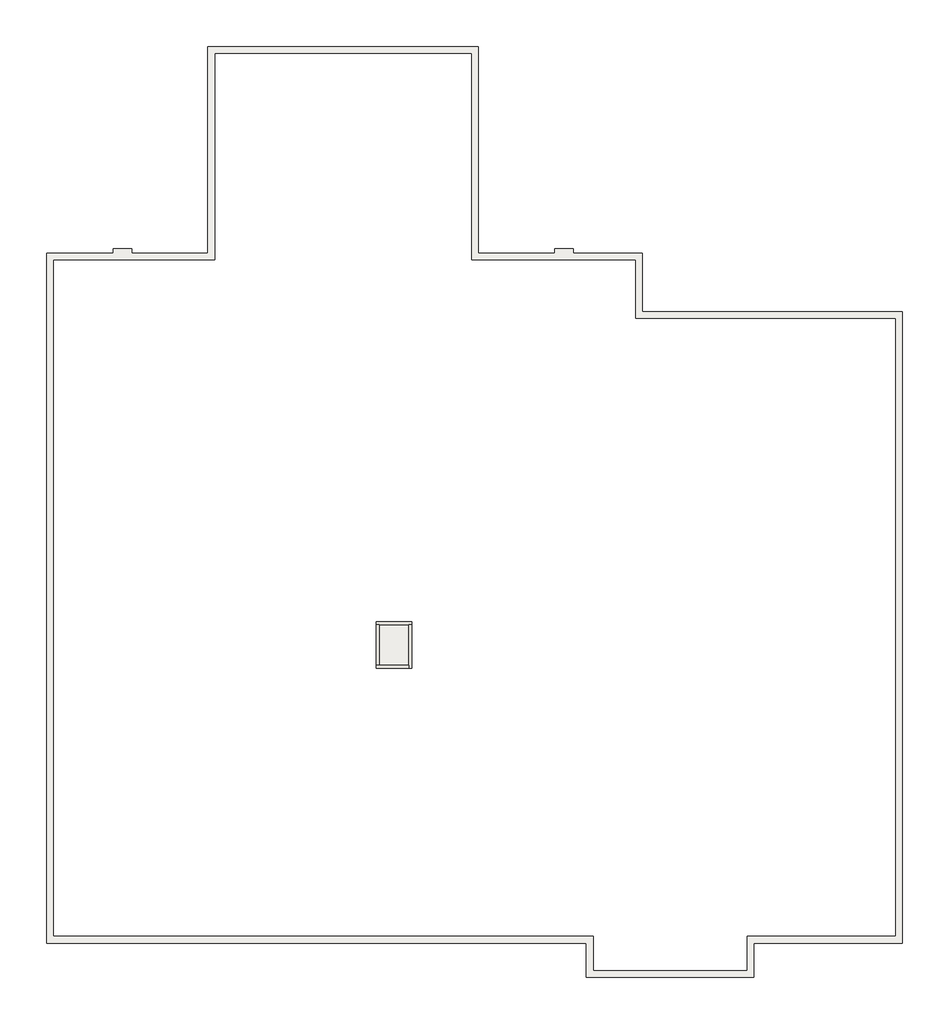
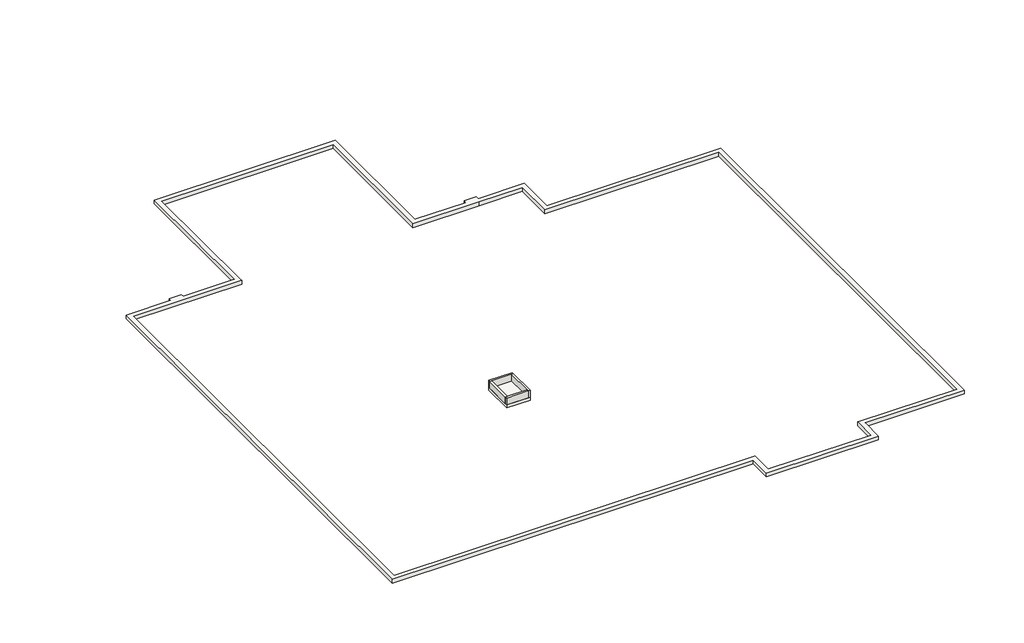
# One storey: 4 walls, 2 slabs.
# Revit data of these elements (continued)
# Project information (continued)
#   PrintManagerSettings = "<PrintManagerDS xmlns=\"http://tempuri.org/PrintManagerDS.xsd\">\n  <xs:schema id=\"PrintManagerDS\" targetNamespace=\"http://tempuri.org/PrintManagerDS.xsd\" xmlns:mstns=\"http://tempuri.org/PrintManagerDS.xsd\" xmlns=\"http://tempuri.org/PrintManagerDS.xsd\" xmlns:xs=\"http://www.w3.org/2001/XMLSchema\" xmlns:msdata=\"urn:schemas-microsoft-com:xml-msdata\" attributeFormDefault=\"qualified\" elementFormDefault=\"qualified\">\n    <xs:element name=\"PrintManagerDS\" msdata:IsDataSet=\"true\" msdata:UseCurrentLocale=\"true\">\n      <xs:complexType>\n        <xs:choice minOccurs=\"0\" maxOccurs=\"unbounded\">\n          <xs:element name=\"DruckEinstellungDT\">\n            <xs:complexType>\n              <xs:sequence>\n                <xs:element name=\"ID\" msdata:DataType=\"System.Guid, mscorlib, Version=4.0.0.0, Culture=neutral, PublicKeyToken=b77a5c561934e089\" msdata:AutoIncrementSeed=\"-1\" msdata:AutoIncrementStep=\"-1\" type=\"xs:string\" minOccurs=\"0\" />\n                <xs:element name=\"Name\" type=\"xs:string\" minOccurs=\"0\" />\n                <xs:element name=\"Beschreibung\" type=\"xs:string\" minOccurs=\"0\" />\n                <xs:element name=\"Kategorie\" type=\"xs:string\" minOccurs=\"0\" />\n                <xs:element name=\"PrinterName\" type=\"xs:string\" minOccurs=\"0\" />\n                <xs:element name=\"PrintToFile\" type=\"xs:boolean\" minOccurs=\"0\" />\n                <xs:element name=\"FileName\" type=\"xs:string\" minOccurs=\"0\" />\n                <xs:element name=\"ColorDepth\" type=\"xs:string\" minOccurs=\"0\" />\n                <xs:element name=\"HiddenLineViews\" type=\"xs:string\" minOccurs=\"0\" />\n                <xs:element name=\"HideCropBoundaries\" type=\"xs:boolean\" minOccurs=\"0\" />\n                <xs:element name=\"HideRefOrWorkPlanes\" type=\"xs:boolean\" minOccurs=\"0\" />\n                <xs:element name=\"HideScopeBoxes\" type=\"xs:boolean\" minOccurs=\"0\" />\n                <xs:element name=\"HideUnreferencedViewTags\" type=\"xs:boolean\" minOccurs=\"0\" />\n                <xs:element name=\"MarginType\" type=\"xs:string\" minOccurs=\"0\" />\n                <xs:element name=\"PageOrientation\" type=\"xs:string\" minOccurs=\"0\" />\n                <xs:element name=\"PaperPlacement\" type=\"xs:string\" minOccurs=\"0\" />\n                <xs:element name=\"PaperSize\" type=\"xs:string\" minOccurs=\"0\" />\n                <xs:element name=\"PaperSource\" type=\"xs:string\" minOccurs=\"0\" />\n                <xs:element name=\"RasterQuality\" type=\"xs:string\" minOccurs=\"0\" />\n                <xs:element name=\"ReplaceHalftoneWithThinLines\" type=\"xs:boolean\" minOccurs=\"0\" />\n                <xs:element name=\"UserDefinedMarginX\" type=\"xs:double\" minOccurs=\"0\" />\n                <xs:element name=\"UserDefinedMarginY\" type=\"xs:double\" minOccurs=\"0\" />\n                <xs:element name=\"ViewLinksInBlue\" type=\"xs:boolean\" minOccurs=\"0\" />\n                <xs:element name=\"Zoom\" type=\"xs:int\" minOccurs=\"0\" />\n                <xs:element name=\"ZoomType\" type=\"xs:string\" minOccurs=\"0\" />\n              </xs:sequence>\n            </xs:complexType>\n          </xs:element>\n          <xs:element name=\"DruckSatzDT\">\n            <xs:complexType>\n              <xs:sequence>\n                <xs:element name=\"ID\" msdata:DataType=\"System.Guid, mscorlib, Version=4.0.0.0, Culture=neutral, PublicKeyToken=b77a5c561934e089\" type=\"xs:string\" minOccurs=\"0\" />\n                <xs:element name=\"PlanID\" type=\"xs:string\" minOccurs=\"0\" />\n                <xs:element name=\"DruckEinstellungID\" msdata:DataType=\"System.Guid, mscorlib, Version=4.0.0.0, Culture=neutral, PublicKeyToken=b77a5c561934e089\" type=\"xs:string\" minOccurs=\"0\" />\n                <xs:element name=\"Name\" type=\"xs:string\" minOccurs=\"0\" />\n                <xs:element name=\"Beschreibung\" type=\"xs:string\" minOccurs=\"0\" />\n                <xs:element name=\"ParameterName\" type=\"xs:string\" minOccurs=\"0\" />\n                <xs:element name=\"File\" type=\"xs:string\" minOccurs=\"0\" />\n                <xs:element name=\"Path\" type=\"xs:string\" minOccurs=\"0\" />\n                <xs:element name=\"GenerateFileName\" type=\"xs:boolean\" minOccurs=\"0\" />\n                <xs:element name=\"Kategorie\" type=\"xs:string\" minOccurs=\"0\" />\n              </xs:sequence>\n            </xs:complexType>\n          </xs:element>\n          <xs:element name=\"DruckJobDT\">\n            <xs:complexType>\n              <xs:sequence>\n                <xs:element name=\"ID\" msdata:DataType=\"System.Guid, mscorlib, Version=4.0.0.0, Culture=neutral, PublicKeyToken=b77a5c561934e089\" type=\"xs:string\" minOccurs=\"0\" />\n                <xs:element name=\"DruckJobGruppeID\" msdata:DataType=\"System.Guid, mscorlib, Version=4.0.0.0, Culture=neutral, PublicKeyToken=b77a5c561934e089\" type=\"xs:string\" minOccurs=\"0\" />\n                <xs:element name=\"DruckSatzID\" msdata:DataType=\"System.Guid, mscorlib, Version=4.0.0.0, Culture=neutral, PublicKeyToken=b77a5c561934e089\" type=\"xs:string\" minOccurs=\"0\" />\n                <xs:element name=\"Anzahl\" type=\"xs:int\" minOccurs=\"0\" />\n              </xs:sequence>\n            </xs:complexType>\n          </xs:element>\n          <xs:element name=\"DruckJobGruppeDT\">\n            <xs:complexType>\n              <xs:sequence>\n                <xs:element name=\"ID\" msdata:DataType=\"System.Guid, mscorlib, Version=4.0.0.0, Culture=neutral, PublicKeyToken=b77a5c561934e089\" type=\"xs:string\" minOccurs=\"0\" />\n                <xs:element name=\"Name\" type=\"xs:string\" minOccurs=\"0\" />\n                <xs:element name=\"Beschreibung\" type=\"xs:string\" minOccurs=\"0\" />\n                <xs:element name=\"JobCount\" msdata:ReadOnly=\"true\" msdata:Expression=\"Count(Child(DruckJobGruppeDT_DruckJobDT).Anzahl)\" type=\"xs:int\" minOccurs=\"0\" />\n                <xs:element name=\"Kategorie\" type=\"xs:string\" minOccurs=\"0\" />\n              </xs:sequence>\n            </xs:complexType>\n          </xs:element>\n          <xs:element name=\"PrintSettingCategories\">\n            <xs:complexType>\n              <xs:sequence>\n                <xs:element name=\"CategoryName\" type=\"xs:string\" minOccurs=\"0\" />\n              </xs:sequence>\n            </xs:complexType>\n          </xs:element>\n          <xs:element name=\"PrintRecordCategories\">\n            <xs:complexType>\n              <xs:sequence>\n                <xs:element name=\"CategoryName\" type=\"xs:string\" />\n              </xs:sequence>\n            </xs:complexType>\n          </xs:element>\n          <xs:element name=\"JobGroupCategories\">\n            <xs:complexType>\n              <xs:sequence>\n                <xs:element name=\"CategoryName\" type=\"xs:string\" />\n              </xs:sequence>\n            </xs:complexType>\n          </xs:element>\n          <xs:element name=\"ExportSettingsDT\">\n            <xs:complexType>\n              <xs:sequence>\n                <xs:element name=\"ID\" msdata:DataType=\"System.Guid, mscorlib, Version=4.0.0.0, Culture=neutral, PublicKeyToken=b77a5c561934e089\" type=\"xs:string\" />\n                <xs:element name=\"Name\" type=\"xs:string\" minOccurs=\"0\" />\n                <xs:element name=\"Description\" type=\"xs:string\" default=\"&quot;&quot;\" minOccurs=\"0\" />\n                <xs:element name=\"Category\" type=\"xs:string\" minOccurs=\"0\" />\n                <xs:element name=\"Type\" type=\"xs:string\" minOccurs=\"0\" />\n                <xs:element name=\"Data\" type=\"xs:string\" minOccurs=\"0\" />\n              </xs:sequence>\n            </xs:complexType>\n          </xs:element>\n          <xs:element name=\"ExportMappingDT\">\n            <xs:complexType>\n              <xs:sequence>\n                <xs:element name=\"ID\" msdata:DataType=\"System.Guid, mscorlib, Version=4.0.0.0, Culture=neutral, PublicKeyToken=b77a5c561934e089\" type=\"xs:string\" />\n                <xs:element name=\"DWG\" msdata:DataType=\"System.Guid, mscorlib, Version=4.0.0.0, Culture=neutral, PublicKeyToken=b77a5c561934e089\" type=\"xs:string\" minOccurs=\"0\" />\n                <xs:element name=\"DWGPath\" type=\"xs:string\" minOccurs=\"0\" />\n                <xs:element name=\"DWGFile\" type=\"xs:string\" minOccurs=\"0\" />\n              </xs:sequence>\n            </xs:complexType>\n          </xs:element>\n          <xs:element name=\"ExportSettingCategories\">\n            <xs:complexType>\n              <xs:sequence>\n                <xs:element name=\"CategoryName\" type=\"xs:string\" />\n              </xs:sequence>\n            </xs:complexType>\n          </xs:element>\n        </xs:choice>\n      </xs:complexType>\n      <xs:unique name=\"Constraint1\">\n        <xs:selector xpath=\".//mstns:DruckEinstellungDT\" />\n        <xs:field xpath=\"mstns:ID\" />\n      </xs:unique>\n      <xs:unique name=\"Constraint2\">\n        <xs:selector xpath=\".//mstns:DruckEinstellungDT\" />\n        <xs:field xpath=\"mstns:Name\" />\n      </xs:unique>\n      <xs:unique name=\"DruckSatzDT_Constraint1\" msdata:ConstraintName=\"Constraint1\">\n        <xs:selector xpath=\".//mstns:DruckSatzDT\" />\n        <xs:field xpath=\"mstns:ID\" />\n      </xs:unique>\n      <xs:unique name=\"DruckJobDT_Constraint1\" msdata:ConstraintName=\"Constraint1\">\n        <xs:selector xpath=\".//mstns:DruckJobDT\" />\n        <xs:field xpath=\"mstns:ID\" />\n      </xs:unique>\n      <xs:unique name=\"DruckJobGruppeDT_Constraint1\" msdata:ConstraintName=\"Constraint1\">\n        <xs:selector xpath=\".//mstns:DruckJobGruppeDT\" />\n        <xs:field xpath=\"mstns:ID\" />\n      </xs:unique>\n      <xs:unique name=\"PrintSettingCategories_Constraint1\" msdata:ConstraintName=\"Constraint1\">\n        <xs:selector xpath=\".//mstns:PrintSettingCategories\" />\n        <xs:field xpath=\"mstns:CategoryName\" />\n      </xs:unique>\n      <xs:unique name=\"PrintRecordCategories_Constraint1\" msdata:ConstraintName=\"Constraint1\" msdata:PrimaryKey=\"true\">\n        <xs:selector xpath=\".//mstns:PrintRecordCategories\" />\n        <xs:field xpath=\"mstns:CategoryName\" />\n      </xs:unique>\n      <xs:unique name=\"JobGroupCategories_Constraint1\" msdata:ConstraintName=\"Constraint1\" msdata:PrimaryKey=\"true\">\n        <xs:selector xpath=\".//mstns:JobGroupCategories\" />\n        <xs:field xpath=\"mstns:CategoryName\" />\n      </xs:unique>\n      <xs:unique name=\"ExportSettingsDT_Constraint1\" msdata:ConstraintName=\"Constraint1\" msdata:PrimaryKey=\"true\">\n        <xs:selector xpath=\".//mstns:ExportSettingsDT\" />\n        <xs:field xpath=\"mstns:ID\" />\n      </xs:unique>\n      <xs:unique name=\"ExportSettingsDT_Constraint2\" msdata:ConstraintName=\"Constraint2\">\n        <xs:selector xpath=\".//mstns:ExportSettingsDT\" />\n        <xs:field xpath=\"mstns:Name\" />\n      </xs:unique>\n      <xs:unique name=\"ExportMappingDT_Constraint1\" msdata:ConstraintName=\"Constraint1\" msdata:PrimaryKey=\"true\">\n        <xs:selector xpath=\".//mstns:ExportMappingDT\" />\n        <xs:field xpath=\"mstns:ID\" />\n      </xs:unique>\n      <xs:unique name=\"ExportSettingCategories_Constraint1\" msdata:ConstraintName=\"Constraint1\" msdata:PrimaryKey=\"true\">\n        <xs:selector xpath=\".//mstns:ExportSettingCategories\" />\n        <xs:field xpath=\"mstns:CategoryName\" />\n      </xs:unique>\n    </xs:element>\n    <xs:annotation>\n      <xs:appinfo>\n        <msdata:Relationship name=\"PrintSettingCategories_DruckEinstellungDT\" msdata:parent=\"PrintSettingCategories\" msdata:child=\"DruckEinstellungDT\" msdata:parentkey=\"CategoryName\" msdata:childkey=\"Kategorie\" />\n        <msdata:Relationship name=\"DruckEinstellungDT_DruckSatzDT\" msdata:parent=\"DruckEinstellungDT\" msdata:child=\"DruckSatzDT
#     \" msdata:parentkey=\"ID\" msdata:childkey=\"DruckEinstellungID\" />\n        <msdata:Relationship name=\"DruckJobGruppeDT_DruckJobDT\" msdata:parent=\"DruckJobGruppeDT\" msdata:child=\"DruckJobDT\" msdata:parentkey=\"ID\" msdata:childkey=\"DruckJobGruppeID\" />\n        <msdata:Relationship name=\"DruckEinstellungDT_PrintRecordCategories\" msdata:parent=\"DruckSatzDT\" msdata:child=\"PrintRecordCategories\" msdata:parentkey=\"Kategorie\" msdata:childkey=\"CategoryName\" />\n        <msdata:Relationship name=\"DruckJobGruppeDT_JobGroupCategories\" msdata:parent=\"DruckJobGruppeDT\" msdata:child=\"JobGroupCategories\" msdata:parentkey=\"Kategorie\" msdata:childkey=\"CategoryName\" />\n        <msdata:Relationship name=\"DruckSatzDT_DruckJobDT\" msdata:parent=\"DruckSatzDT\" msdata:child=\"DruckJobDT\" msdata:parentkey=\"ID\" msdata:childkey=\"DruckSatzID\" />\n        <msdata:Relationship name=\"DruckSatzDT_ExportMappingDT\" msdata:parent=\"DruckSatzDT\" msdata:child=\"ExportMappingDT\" msdata:parentkey=\"ID\" msdata:childkey=\"ID\" />\n        <msdata:Relationship name=\"ExportSettingsDT_ExportSettingCategories\" msdata:parent=\"ExportSettingCategories\" msdata:child=\"ExportSettingsDT\" msdata:parentkey=\"CategoryName\" msdata:childkey=\"Category\" />\n      </xs:appinfo>\n    </xs:annotation>\n  </xs:schema>\n  <PrintRecordCategories>\n    <CategoryName>&lt;Keine&gt;</CategoryName>\n  </PrintRecordCategories>\n  <JobGroupCategories>\n    <CategoryName>&lt;Keine&gt;</CategoryName>\n  </JobGroupCategories>\n</PrintManagerDS>"
#   5D Template Project Version Info  = "AAEAAAD/////AQAAAAAAAAAMAgAAAE5UZW1wbGF0ZVZlcnNpb25JbmZvMjAxMywgVmVyc2lvbj0xLjAuMC4wLCBDdWx0dXJlPW5ldXRyYWwsIFB1YmxpY0tleVRva2VuPW51bGwFAQAAACpzdHJhYmFnLnp0LlRlbXBsYXRlVmVyc2lvbkluZm8uVmVyc2lvbkluZm8HAAAAD3Zlck1ham9yUmVsZWFzZQ92ZXJNaW5vclJlbGVhc2UNdmVyUGF0Y2hMZXZlbAxyZXZpdFZlcnNpb24KY3VzdG9tZXJJZAtyZWxlYXNlRGF0ZRFicmFuZGluZ1RpbWVTdGFtcAAAAAAAAAAICAgICA0NAgAAAAEAAAAAAAAAAAAAAN0HAADtAwAAAICidKSRzwhNrtviDpLPiAs="
#   Kostenstelle = "570-XXX"
#   Bauherr = "Firmenbezeichnung Bauherr\nZusatz XY GmbH\nAngabe der Strasse 34\n99999 Ortschaft"
#   Projektmanagement = "Firmenbezeichnung Projektmanagement\nZusatz XY GmbH\nAngabe der Strasse 34\n99999 Ortschaft"
#   Ausführungsplanung = "Firmenbezeichnung Ausführungsplanung\nZusatz XY GmbH\nAngabe der Strasse 34\n99999 Ortschaft"
#   Entwurfsplanung = "Firmenbezeichnung Entwurfsplanung\nZusatz XY GmbH\nAngabe der Strasse 34\n99999 Ortschaft"
#   Generalunternehmer = "Ed. Züblin AG\nAlbstadtweg 3\n70567 Stuttgart\nTel. +49 711 7883-0"
#   Planverfasser (Firma) = "Ed. Züblin AG\nAlbstadtweg 3\n70567 Stuttgart\nTel. +49 711 7883-0"
#   Projektausgabedatum = "Projekt Datum"
#   Projektstatus = "Projektstatus"
#   Auftraggeber = "Direktion"
#   Projektadresse = "5D-MUSTERSTRASSE 00, 99999 MUSTERSTADT"
#   Projektname = "Z3_Rohbau"
#   Projektnummer = "abcd-12-DD"
#   BimM_Tools_Initialized = "20100210"
#   bimmTools_bimmTool_Init = "20131021"
#   bimmTools_RFT_Init = "20100112"
#   magiParamsCreated = "2012.11"
#   AreaCalculationInternationalBuildNumber = "ZgA=BAAAAA==2013BgFlAAAAAQgAAAABAQAAAAYBZAAAAAHdBwAABAQAAAABZQIAAAcH0"
#   5dki Contentversion = "2.0"
#   5dfas Contentversion = "1.0"
#   5dsfb Contentversion = "1.0"
# Grids (mm)
#   "1": line (0, 38153.54) -> (0, -20876.403)
#   "2": line (3117, 1567.012) -> (3117, -20876.403)
#   "3": line (7617, 6850) -> (7617, -20876.403)
#   "4": line (12117, 6850) -> (12117, -20876.403)
#   "5": line (16617, 6850) -> (16617, -20876.403)
#   "6": line (21117, 6850) -> (21117, -20876.403)
#   "7": line (25617, 6850) -> (25617, -20876.403)
#   "8": line (30117, 6850) -> (30117, -20876.403)
#   "9": line (34617, 6850) -> (34617, -20876.403)
#   "10": line (39117, 6850) -> (39117, -20876.403)
#   "11": line (43617, 12067.012) -> (43617, -20876.403)
#   "12": line (48117, 3067.012) -> (48117, -20876.403)
#   "13": line (49734, 21562.405) -> (49734, -20876.403)
#   "2-1": line (4405, 24067.012) -> (4405, -19865.202)
#   "2-2": line (6865, 6850) -> (6865, -19865.202)
#   "4-1": line (15242.001, 6850) -> (15242.001, -19865.202)
#   "7-1": line (27767, 6850) -> (27767, -19865.202)
#   "7-2": line (30517, 6850) -> (30517, -19865.202)
#   "9-1": line (35119.999, 6850) -> (35119.999, -19865.202)
#   "10-1": line (41419.999, 6850) -> (41419.999, -19865.202)
#   "11-1": line (44329, 6850) -> (44329, -19865.202)
#   "A": line (76532.912, 0) -> (-6403.276, 0)
#   "B": line (3117, 1567.012) -> (-6403.276, 1567.012)
#   "C": line (4405, 6067.012) -> (-6403.276, 6067.012)
#   "D": line (76532.912, 10567.012) -> (-6403.276, 10567.012)
#   "E": line (15205.86, 15067.012) -> (-6403.276, 15067.012)
#   "F": line (11966.08, 19567.012) -> (-6403.276, 19567.012)
#   "G": line (4405, 24067.012) -> (-6403.276, 24067.012)
#   "H": line (899.272, 28567.012) -> (-6403.276, 28567.012)
#   "I": line (-6350.348, 32762.643) -> (16649.125, 28921.991)
#   "C-1": line (75979.999, 6850) -> (-4869.274, 6850)
#   "L": line (76532.912, 3067.012) -> (48117, 3067.012)
#   "M": line (76532.912, 7567.012) -> (43617, 7567.012)
#   "N": line (76532.912, 12067.012) -> (43617, 12067.012)
#   "O": line (76532.912, 15067.012) -> (46346.98, 15067.012)
#   "P": line (56099.768, 16087.731) -> (36260.662, 19400.637)
#   "Q": line (52187.753, 22227.766) -> (22325.754, 16927.13)
#   "K": line (22325.754, 16927.13) -> (8861.069, 35629.353)
#   "J": line (905.356, 34930.174) -> (18445.639, 10567.012)
#   "14": line (899.272, 28567.012) -> (2431.299, 37741.445)
#   "15": line (5822.756, 30729.872) -> (6869.839, 37000.258)
#   "17": line (9531.776, 25620.01) -> (11308.38, 36259.072)
#   "18": line (16915.158, 35322.804) -> (13285.676, 29483.649)
#   "19": line (11810.999, 22666.315) -> (21182.49, 29413.33)
#   "20": line (14440.253, 19014.326) -> (23811.744, 25761.341)
#   "21": line (17069.506, 15362.337) -> (26440.997, 22109.351)
#   "22": line (25037.995, 12277.662) -> (23041.496, 23525.23)
#   "23": line (29404.461, 13426.23) -> (27472.236, 24311.707)
#   "24": line (33899.473, 13850.618) -> (31902.975, 25098.184)
#   "25": line (37049.216, 14030.16) -> (38617.163, 23419.701)
#   "26": line (41487.757, 13288.974) -> (43055.704, 22678.514)
#   "27": line (46346.98, 15067.014) -> (47494.245, 21937.328)
#   "UC": line (76532.912, -4330) -> (-6403.276, -4330)
#   "UB": line (76532.912, -11930) -> (-6403.276, -11930)
#   "UA": line (76532.912, -16280) -> (-6403.276, -16280)
#   "UD": line (17970, 25643.928) -> (-6403.276, 25643.928)
#   "UF": line (25570, 37335.574) -> (-6403.276, 37335.574)
#   "UG": line (13620, 41539.528) -> (-6403.276, 41539.528)
#   "UH": line (54022.494, 42635.573) -> (-6403.276, 42635.573)
#   "UI": line (54022.494, 47935.573) -> (-6403.276, 47935.573)
#   "UJ": line (54022.494, 53235.573) -> (-6403.276, 53235.573)
#   "UK": line (54022.494, 58975.928) -> (-6403.276, 58975.928)
#   "U6": line (13620, 24235.573) -> (13620, 63763.457)
#   "U7": line (17970, 24235.573) -> (17970, 63763.457)
#   "U8": line (25570, 24235.573) -> (25570, 63763.457)
#   "U9": line (29670, 24235.573) -> (29670, 63763.457)
#   "U10": line (34470, 24235.573) -> (34470, 63763.457)
#   "U11": line (36120, 36635.573) -> (36120, 63763.457)
#   "UM": line (76532.912, 29535.573) -> (-6403.276, 29535.573)
#   "UN": line (76532.912, 36635.573) -> (36120, 36635.573)
#   "UL": line (76532.912, 24235.573) -> (25570, 24235.573)
#   "U1": line (52619.999, -4323.869) -> (52619.999, -22332.496)
#   "U2": line (57919.999, -4323.869) -> (57919.999, -22332.496)
#   "U3": line (63219.999, -4323.869) -> (63219.999, -22332.496)
#   "U4": line (68519.999, -4323.869) -> (68519.999, -22332.496)
#   "U5": line (71829.999, 37785.574) -> (71829.999, -22332.496)
#   "U12": line (42046.606, 37785.574) -> (42046.606, 24263.521)
#   "U13": line (46520, 37785.574) -> (46520, 24263.521)
#   "U14": line (50970, 37785.574) -> (50970, 24263.521)
#   "U15": line (58569.999, 37785.574) -> (58569.999, 0)
#   "U16": line (63729.999, 37785.574) -> (63729.999, 0)
# Type "5dki Aufzugsunterfahrt Bopla 40cm C40/50"
#   cpiComponentType = "Foundation_Slab"
#   cpiFitMatchKey = "5D-KI-STB-OB-FU-AUB"
#   5d Materialgüte = "C40/50"
#   5dki WU = no
#   Layers, outside or top first: 0.400 m "5d Beton - Stahlbeton" (function 1)
# Type "5dki Streifenfundament 50cm C100/115"
#   cpiComponentType = "Foundation"
#   cpiFitMatchKey = "5D-KI-STB-OB-FU-SF"
#   5d Materialgüte = "C100/115"
#   5dki Bewehrung Stab kg pro m3 = 0
#   5dki Bewehrung Liste kg pro m3 = 0
#   5dki Bewehrung Matte kg pro m3 = 0
#   5dki WU = no
#   Layers, outside or top first: 0.500 m "5d Beton - Stahlbeton" (function 1)
# Type "5dki Aufzugsunterfahrt STB-Wand 25cm C40/50"
#   Type Comments = ""
#   Description = ""
#   cpiComponentType = "Wall"
#   cpiFitMatchKey = "5D-KI-STB-OB-FU-AUW"
#   5d Materialgüte = "C40/50"
#   Filter Tragend / Nichttragend = yes
#   Layers, outside or top first: 0.250 m "5d Beton - Stahlbeton" (function 1)
# Element 1 (IfcSlab, "5dki Aufzugsunterfahrt Bopla 40cm C40/50")
#   000_080_030_Geschoß = "02_FU"
#   Height Offset From Level = 0.000 m
#   built-in parameter 1001954 = 1
#   Phase Created = Neu
#   Materials on its faces: "5d Beton - Stahlbeton"
# Element 2 (IfcSlab, "5dki Streifenfundament 50cm C100/115")
#   built-in parameter 1001955 = 3.14159 (stored number, unit not read)
#   Height Offset From Level = 0.500 m
#   built-in parameter 1001954 = 1
#   5dki Sauberkeitsschicht = yes
#   5dki Trennlage = yes
#   5dki gekrümmt = no
#   5dki Abzug Sauberkeitsschicht BoPla = yes
#   Phase Created = Neu
#   Materials on its faces: "5d Beton - Stahlbeton"
# Element 3 (IfcWall, "5dki Aufzugsunterfahrt STB-Wand 25cm C40/50")
#   Comments = ""
#   000_080_030_Geschoß = "02_FU"
#   Top Offset = 0.000 m
#   Base Offset = 0.000 m
#   wall height = 0.900 m
#   Phase Created = Neu
#   Base Constraint = 02_FU_OKFU_-5,10__Aufzug
#   Top Constraint = 02_FU_OKRD_-4,20
#   Materials on its faces: "5d Beton - Stahlbeton"
# Elements 4, 5, 6 (IfcWall, "5dki Aufzugsunterfahrt STB-Wand 25cm C40/50")
#   000_080_030_Geschoß = "02_FU"
#   Top Offset = 0.000 m
#   Base Offset = 0.000 m
#   wall height = 0.900 m
#   Phase Created = Neu
#   Base Constraint = 02_FU_OKFU_-5,10__Aufzug
#   Top Constraint = 01_UG_OKFB_-4,20
#   Materials on its faces: "5d Beton - Stahlbeton"
# Materials
#   "5d Beton - Stahlbeton": class "5dki", colour RGB 200 200 200, transparency 0, Cost = 0
